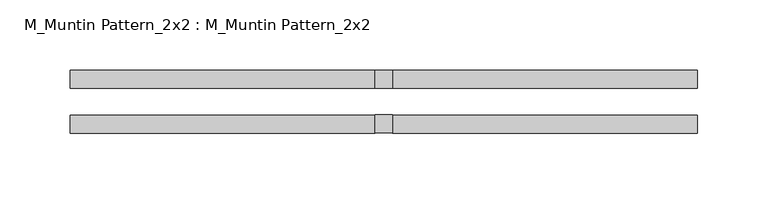
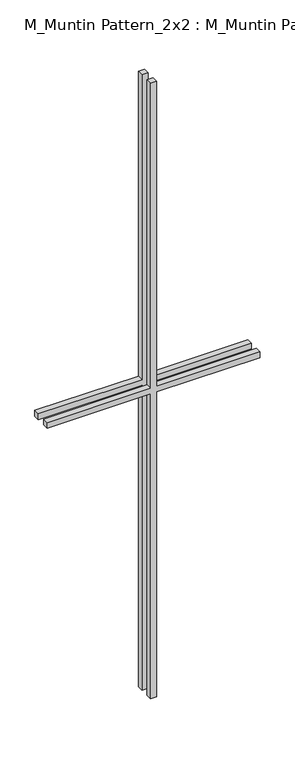
"""IFC4 building model written with IfcOpenShell, lengths in millimetres: proxy geometry, M_Muntin Pattern_2x2 : M_Muntin Pattern_2x2."""

from ifc_helpers import new_model, si_unit, frame, origin, place, context, project, spatial, polyline, outline, extrude, source, transform, mapped, element, save


def m_muntin_pattern_2x2_m_muntin_pattern_2x2_86194ec4(model_context):
    return source(origin(), model_context, "Body", "SweptSolid", [
        extrude(outline(polyline([(686.5, -6.35), (686.5, -223.0), (673.8, -223.0), (673.8, -6.35), (0.0, -6.35), (0.0, 6.35), (673.8, 6.35), (673.8, 223.0), (686.5, 223.0), (686.5, 6.35), (1360.3, 6.35), (1360.3, -6.35), (686.5, -6.35)])), frame((0.0, -22.225, 0.0), z_axis=(0.0, 1.0, 0.0), x_axis=(0.0, 0.0, 1.0)), (0.0, 0.0, 1.0), 12.7),
        extrude(outline(polyline([(686.5, -6.35), (686.5, -223.0), (673.8, -223.0), (673.8, -6.35), (0.0, -6.35), (0.0, 6.35), (673.8, 6.35), (673.8, 223.0), (686.5, 223.0), (686.5, 6.35), (1360.3, 6.35), (1360.3, -6.35), (686.5, -6.35)])), frame((0.0, 9.525, 0.0), z_axis=(0.0, 1.0, 0.0), x_axis=(0.0, 0.0, 1.0)), (0.0, 0.0, 1.0), 12.7),
    ])


if __name__ == "__main__":
    model = new_model("IFC4")
    model_context = context("Model", 3, world=origin())
    ifc_project = project(units=[si_unit("LENGTHUNIT", "METRE", prefix="MILLI")], contexts=[model_context])
    site = spatial("IfcSite", under=ifc_project)
    building = spatial("IfcBuilding", under=site)
    placement = place(None, origin())
    m_muntin_pattern_2x2_m_muntin_pattern_2x2_shape = m_muntin_pattern_2x2_m_muntin_pattern_2x2_86194ec4(model_context)
    element("IfcBuildingElementProxy", 1, Name="M_Muntin Pattern_2x2 : M_Muntin Pattern_2x2", ObjectType="M_Muntin Pattern_2x2 : M_Muntin Pattern_2x2", at=placement, inside=building, context=model_context, shape_type="MappedRepresentation", body=[
        mapped(m_muntin_pattern_2x2_m_muntin_pattern_2x2_shape, transform((0.0, 0.0, 0.0), x_axis=(1.0, 0.0, 0.0), y_axis=(0.0, 1.0, 0.0), z_axis=(0.0, 0.0, 1.0))),
    ])
    save(model, "model.ifc")

# Revit data of these elements
# Type "M_Muntin Pattern_2x2 : M_Muntin Pattern_2x2"
#   Width [instance default] = 1200 mm
#   Thickness = 12.7 mm
#   Height [instance default] = 1200 mm
#   Distance = 19.05 mm
#   Interior Material [instance default] = none
#   Exterior Material [instance default] = none
#   Default Elevation = 0
# Element 1 (IfcBuildingElementProxy, "M_Muntin Pattern_2x2 : M_Muntin Pattern_2x2")
#   Width = 446 mm
#   Height = 1360.3 mm
#   Interior Material = Wood - Stained
#   Exterior Material = Clad - White
#   Materials on its faces: "Clad - White", "Wood - Stained"
# Materials
#   "Clad - White": class "Wood", colour RGB 242 242 238, transparency 0, Cost = 0
#   "Wood - Stained": class "Wood", colour RGB 227 170 128, transparency 0, Cost = 0
